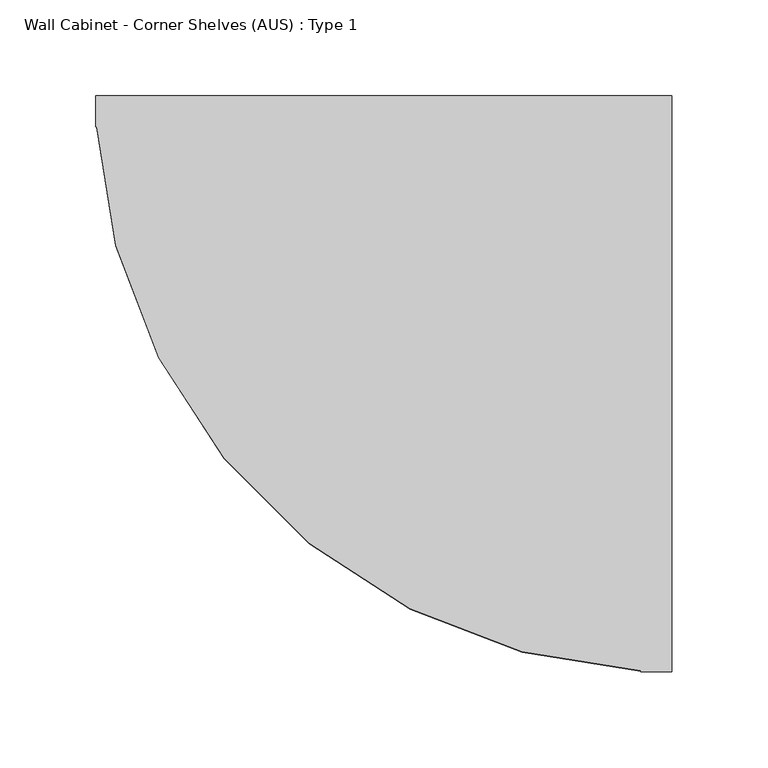
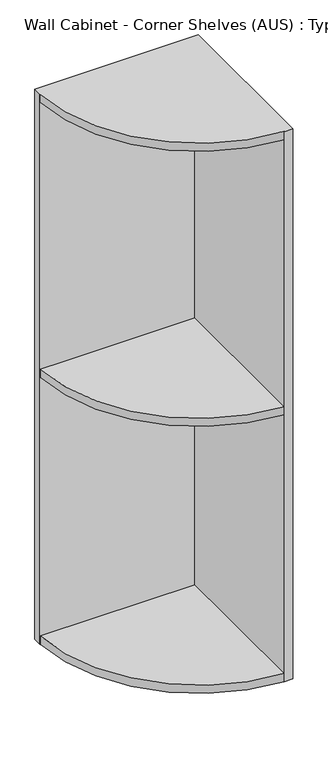
"""IFC4 building model written with IfcOpenShell, lengths in millimetres: furniture geometry, Wall Cabinet - Corner Shelves (AUS) : Type 1."""

from ifc_helpers import new_model, si_unit, frame, origin, place, context, project, spatial, circle_curve, source, transform, mapped, element, save
from ifc_brep_helpers import plane_surface, cylinder_surface, advanced_brep


def wall_cabinet_corner_shelves_aus_type_1_ea0bf300(model_context):
    return source(origin(), model_context, "Body", "AdvancedBrep", [
        advanced_brep(
        [(-25.0, -168.6180748, 2566.8), (-25.0, -184.6180748, 2566.8), (-24.5730295, -184.6180748, 2566.8), (259.0, -468.1911042, 2566.8), (259.0, -468.6180748, 2566.8), (275.0, -468.6180748, 2566.8), (275.0, -168.6180748, 2566.8), (-24.5730295, -184.6180748, 2550.8), (259.0, -184.6180748, 2550.8), (259.0, -468.1911042, 2550.8), (275.0, -168.6180748, 2033.4), (275.0, -168.6180748, 2017.4), (275.0, -168.6180748, 1516.0), (275.0, -168.6180748, 1500.0), (-25.0, -168.6180748, 1500.0), (-25.0, -168.6180748, 1516.0), (-25.0, -168.6180748, 2017.4), (-25.0, -168.6180748, 2033.4), (275.0, -468.6180748, 2033.4), (275.0, -468.6180748, 2017.4), (275.0, -468.6180748, 1516.0), (275.0, -468.6180748, 1500.0), (259.0, -468.6180748, 1500.0), (259.0, -468.1911042, 1500.0), (-24.5730295, -184.6180748, 1500.0), (-25.0, -184.6180748, 1500.0), (259.0, -184.6180748, 2033.4), (259.0, -468.1911042, 2033.4), (259.0, -468.1911042, 2017.4), (259.0, -184.6180748, 2017.4), (259.0, -184.6180748, 1516.0), (259.0, -468.1911042, 1516.0), (-24.5730295, -184.6180748, 1516.0), (-24.5730295, -184.6180748, 2017.4), (-24.5730295, -184.6180748, 2033.4)],
        [
            (0, 1),
            (1, 2),
            (2, 3, circle_curve(frame((275.0, -168.6180748, 2566.8), z_axis=(0.0, 0.0, 1.0), x_axis=(0.0, -1.0, 0.0)), 300.0)),
            (3, 4),
            (4, 5),
            (5, 6),
            (6, 0),
            (7, 8),
            (8, 9),
            (9, 7, circle_curve(frame((275.0, -168.6180748, 2550.8), z_axis=(0.0, 0.0, -1.0), x_axis=(0.0, -1.0, 0.0)), 300.0)),
            (6, 10),
            (10, 11),
            (11, 12),
            (12, 13),
            (13, 14),
            (14, 15),
            (15, 16),
            (16, 17),
            (17, 0),
            (5, 18),
            (18, 19),
            (19, 20),
            (20, 21),
            (21, 13),
            (2, 7),
            (9, 3),
            (21, 22),
            (22, 23),
            (23, 24, circle_curve(frame((275.0, -168.6180748, 1500.0), z_axis=(0.0, 0.0, -1.0), x_axis=(0.0, -1.0, 0.0)), 300.0)),
            (24, 25),
            (25, 14),
            (4, 22),
            (8, 26),
            (26, 27),
            (27, 28),
            (28, 29),
            (29, 30),
            (30, 31),
            (31, 23),
            (24, 32),
            (32, 30),
            (29, 33),
            (33, 34),
            (34, 26),
            (1, 25),
            (34, 27, circle_curve(frame((275.0, -168.6180748, 2033.4), z_axis=(0.0, 0.0, 1.0), x_axis=(0.0, -1.0, 0.0)), 300.0)),
            (28, 33, circle_curve(frame((275.0, -168.6180748, 2017.4), z_axis=(0.0, 0.0, -1.0), x_axis=(0.0, -1.0, 0.0)), 300.0)),
            (32, 31, circle_curve(frame((275.0, -168.6180748, 1516.0), z_axis=(0.0, 0.0, 1.0), x_axis=(0.0, -1.0, 0.0)), 300.0)),
        ],
        [
            plane_surface(frame((275.0, -168.6180748, 2566.8), z_axis=(0.0, 0.0, 1.0), x_axis=(1.0, 0.0, 0.0))),
            plane_surface(frame((275.0, -168.6180748, 2550.8), z_axis=(0.0, 0.0, -1.0), x_axis=(-1.0, 0.0, 0.0))),
            plane_surface(frame((-25.0, -168.6180748, 2566.8), z_axis=(0.0, 1.0, 0.0), x_axis=(0.0, 0.0, -1.0))),
            plane_surface(frame((275.0, -168.6180748, 2566.8), z_axis=(1.0, 0.0, 0.0), x_axis=(0.0, 0.0, -1.0))),
            cylinder_surface(frame((275.0, -168.6180748, 2550.8), z_axis=(0.0, 0.0, 1.0), x_axis=(0.0, -1.0, 0.0)), 300.0),
            plane_surface(frame((259.0, -468.6180748, 1500.0), z_axis=(0.0, 0.0, -1.0), x_axis=(1.0, 0.0, 0.0))),
            plane_surface(frame((275.0, -468.6180748, 2566.8), z_axis=(0.0, -1.0, 0.0), x_axis=(0.0, 0.0, -1.0))),
            plane_surface(frame((259.0, -468.6180748, 2566.8), z_axis=(-1.0, 0.0, 0.0), x_axis=(0.0, 0.0, -1.0))),
            plane_surface(frame((259.0, -184.6180748, 2566.8), z_axis=(0.0, -1.0, 0.0), x_axis=(0.0, 0.0, -1.0))),
            plane_surface(frame((-25.0, -184.6180748, 2566.8), z_axis=(-1.0, 0.0, 0.0), x_axis=(0.0, 0.0, -1.0))),
            plane_surface(frame((275.0, -168.6180748, 2033.4), z_axis=(0.0, 0.0, 1.0), x_axis=(1.0, 0.0, 0.0))),
            plane_surface(frame((275.0, -168.6180748, 2017.4), z_axis=(0.0, 0.0, -1.0), x_axis=(-1.0, 0.0, 0.0))),
            cylinder_surface(frame((275.0, -168.6180748, 2017.4), z_axis=(0.0, 0.0, 1.0), x_axis=(0.0, -1.0, 0.0)), 300.0),
            plane_surface(frame((275.0, -168.6180748, 1516.0), z_axis=(0.0, 0.0, 1.0), x_axis=(1.0, 0.0, 0.0))),
            cylinder_surface(frame((275.0, -168.6180748, 1500.0), z_axis=(0.0, 0.0, 1.0), x_axis=(0.0, -1.0, 0.0)), 300.0),
        ],
        [
            (0, [[1, 2, 3, 4, 5, 6, 7]]),
            (1, [[8, 9, 10]]),
            (2, [[11, 12, 13, 14, 15, 16, 17, 18, 19, -7]]),
            (3, [[20, 21, 22, 23, 24, -14, -13, -12, -11, -6]]),
            (4, [[25, -10, 26, -3]]),
            (5, [[27, 28, 29, 30, 31, -15, -24]]),
            (6, [[32, -27, -23, -22, -21, -20, -5]]),
            (7, [[-4, -26, -9, 33, 34, 35, 36, 37, 38, 39, -28, -32]]),
            (8, [[-30, 40, 41, -37, 42, 43, 44, -33, -8, -25, -2, 45]]),
            (9, [[-19, -18, -17, -16, -31, -45, -1]]),
            (10, [[-34, -44, 46]]),
            (11, [[-42, -36, 47]]),
            (12, [[-43, -47, -35, -46]]),
            (13, [[-38, -41, 48]]),
            (14, [[-39, -48, -40, -29]]),
        ],
    ),
    ])


if __name__ == "__main__":
    model = new_model("IFC4")
    model_context = context("Model", 3, world=origin())
    ifc_project = project(units=[si_unit("LENGTHUNIT", "METRE", prefix="MILLI")], contexts=[model_context])
    site = spatial("IfcSite", under=ifc_project)
    building = spatial("IfcBuilding", under=site)
    placement = place(None, origin())
    wall_cabinet_corner_shelves_aus_type_1_shape = wall_cabinet_corner_shelves_aus_type_1_ea0bf300(model_context)
    element("IfcFurniture", 1, ObjectType="Wall Cabinet - Corner Shelves (AUS) : Type 1", at=placement, inside=building, context=model_context, shape_type="MappedRepresentation", body=[
        mapped(wall_cabinet_corner_shelves_aus_type_1_shape, transform((0.0, 0.0, 0.0), x_axis=(1.0, 0.0, 0.0), y_axis=(0.0, 1.0, 0.0), z_axis=(0.0, 0.0, 1.0))),
    ])
    save(model, "model.ifc")

# Revit data of these elements
# Type "Wall Cabinet - Corner Shelves (AUS) : Type 1"
#   COBie.Type.CreatedBy = "doug.wood@us.ibm.com"
#   COBie.Type.CreatedOn = "2016-04-14T02:07:23"
#   COBie.Type.Name = "Casework_Wall Cabinet - Corner Shelves (AUS)_Type 1"
#   COBie.Type.Category = "n/a"
#   COBie.Type.Description = "Wall Cabinet - Corner Shelves (AUS)_Type 1"
#   COBie.Type.Manufacturer = ""
#   COBie.Type.ModelNumber = ""
#   COBie.Type.ReplacementCost = 0
#   Width [instance default] = 0' - 11.81102"
#   Height [instance default] = 1' - 11.62205"
#   Depth [instance default] = 0' - 11.81102"
#   COBie.Type = no
#   Show Outline [instance default] = no
#   Show Hidden [instance default] = yes
#   Assembly Code = ""
# Element 1 (IfcFurniture, "Wall Cabinet - Corner Shelves (AUS) : Type 1")
#   Height = 3' - 6"
